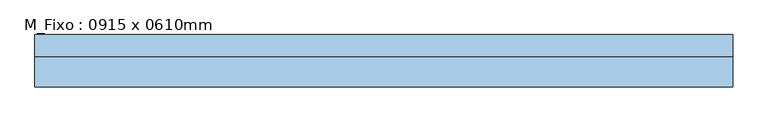
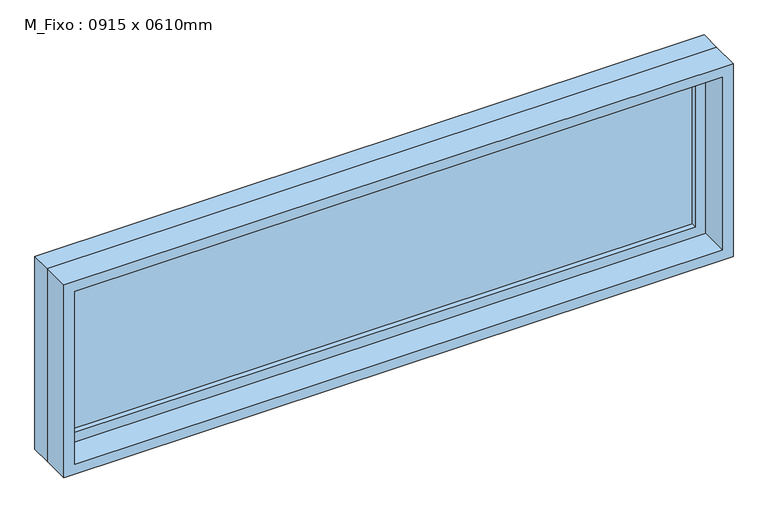
"""IFC4 building model written with IfcOpenShell, lengths in millimetres: window geometry, M_Fixo : 0915 x 0610mm."""

from ifc_helpers import new_model, si_unit, frame, origin, place, context, project, spatial, polyline, outline, extrude, source, transform, mapped, element, save


def m_fixo_0915_x_0610mm_568dc35f(model_context):
    return source(origin(), model_context, "Body", "SweptSolid", [
        extrude(outline(polyline([(-937.0, 53.0), (937.0, 53.0), (937.0, 41.0), (-937.0, 41.0), (-937.0, 53.0)])), frame((0.0, 0.0, 2063.0), z_axis=(0.0, 0.0, 1.0), x_axis=(1.0, 0.0, 0.0)), (0.0, 0.0, 1.0), 484.0),
        extrude(outline(polyline([(2591.0, -981.0), (2019.0, -981.0), (2019.0, 981.0), (2591.0, 981.0), (2591.0, -981.0)]), holes=[polyline([(2547.0, -937.0), (2547.0, 937.0), (2063.0, 937.0), (2063.0, -937.0), (2547.0, -937.0)])]), frame((0.0, 25.0, 0.0), z_axis=(0.0, 1.0, 0.0), x_axis=(0.0, 0.0, 1.0)), (0.0, 0.0, 1.0), 44.0),
        extrude(outline(polyline([(2610.0, -1000.0), (2000.0, -1000.0), (2000.0, 1000.0), (2610.0, 1000.0), (2610.0, -1000.0)]), holes=[polyline([(2591.0, -981.0), (2591.0, 981.0), (2019.0, 981.0), (2019.0, -981.0), (2591.0, -981.0)])]), frame((0.0, 25.0, 0.0), z_axis=(0.0, 1.0, 0.0), x_axis=(0.0, 0.0, 1.0)), (0.0, 0.0, 1.0), 63.0),
        extrude(outline(polyline([(2610.0, -1000.0), (2000.0, -1000.0), (2000.0, 1000.0), (2610.0, 1000.0), (2610.0, -1000.0)]), holes=[polyline([(2578.0, -968.0), (2578.0, 968.0), (2032.0, 968.0), (2032.0, -968.0), (2578.0, -968.0)])]), frame((0.0, -62.0, 0.0), z_axis=(0.0, 1.0, 0.0), x_axis=(0.0, 0.0, 1.0)), (0.0, 0.0, 1.0), 87.0),
    ])


if __name__ == "__main__":
    model = new_model("IFC4")
    model_context = context("Model", 3, world=origin())
    ifc_project = project(units=[si_unit("LENGTHUNIT", "METRE", prefix="MILLI")], contexts=[model_context])
    site = spatial("IfcSite", under=ifc_project)
    building = spatial("IfcBuilding", under=site)
    placement = place(None, origin())
    m_fixo_0915_x_0610mm_shape = m_fixo_0915_x_0610mm_568dc35f(model_context)
    element("IfcWindow", 1, ObjectType="M_Fixo : 0915 x 0610mm", at=placement, inside=building, context=model_context, shape_type="MappedRepresentation", body=[
        mapped(m_fixo_0915_x_0610mm_shape, transform((0.0, 0.0, 0.0), x_axis=(1.0, 0.0, 0.0), y_axis=(0.0, 1.0, 0.0), z_axis=(0.0, 0.0, 1.0))),
    ])
    save(model, "model.ifc")

# Revit data of these elements
# Type "M_Fixo : 0915 x 0610mm"
#   Type Mark = "14"
#   Construction Type Id = "GSP4R"
#   Analytic Construction = "Vidraça única Pilkington 1/8 pol"
#   Visual Light Transmittance = 0.9
#   Thermal Resistance (R) = 0.271106 (m²·K)/W
#   Solar Heat Gain Coefficient = 0.78
#   Heat Transfer Coefficient (U) = 3.6886 W/(m²·K)
#   Height = 0.61 m
#   Altura-padrão do peitoril = 2.00 m
#   Width = 2.00 m
#   Janela aplicada = 0.019 m
#   Define Thermal Properties by = 1
#   Material da estrutura externa = Caixilho
#   Material da estrutura interna = Caixilho
#   Material do painel de vidro = Vidro
#   Caixilho = Caixilho
#   Wall Closure = (empty or 0)
# Element 1 (IfcWindow, "M_Fixo : 0915 x 0610mm")
#   Materials on its faces: "Caixilho", "Vidro"
# Materials
#   "Caixilho": class "Madeira", colour RGB 224 178 126, transparency 0, Cost = 0
#   "Vidro": class "Vidro", colour RGB 0 128 192, transparency 0.9, Description = "Vidro de sílica", Cost = 0
